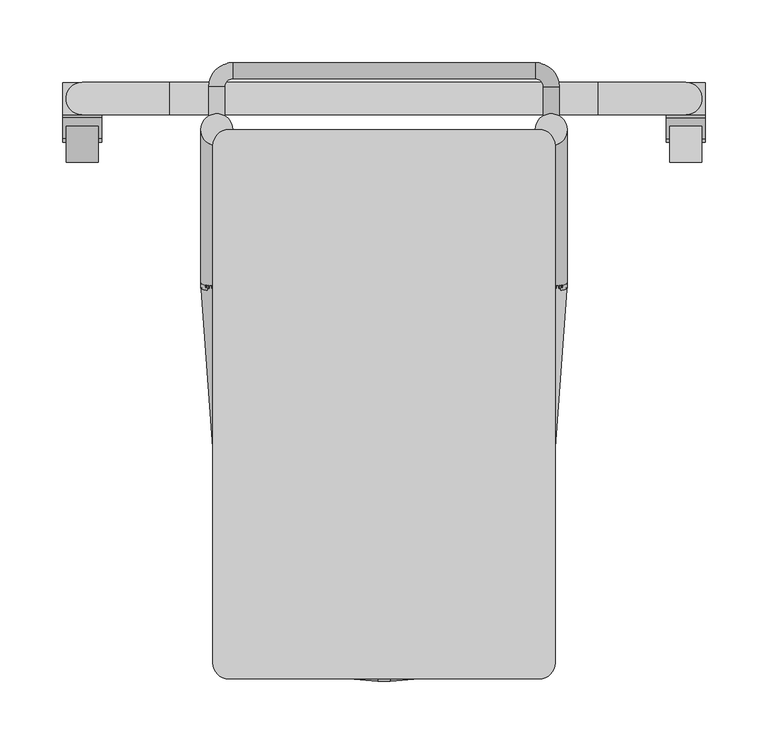
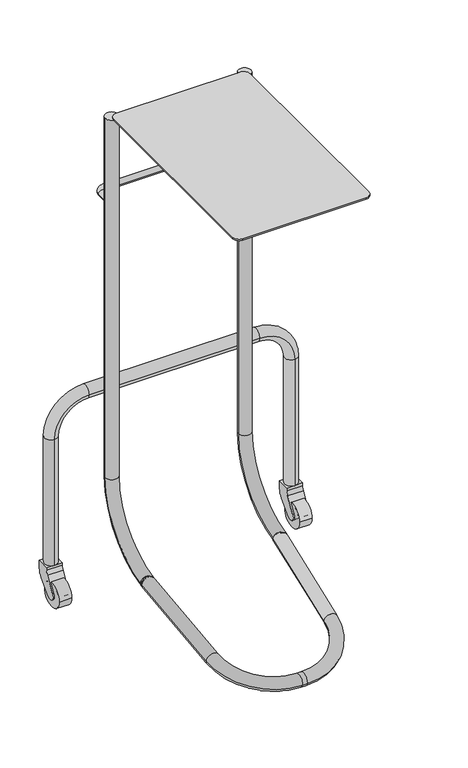
"""IFC4 building model written with IfcOpenShell, lengths in millimetres: proxy geometry, M8810 - Stand, Mayo : M8810 - Stand, Mayo."""

import ifcopenshell
import ifcopenshell.guid

model = None  # the IFC model being written
_history = None  # IfcOwnerHistory: only IFC2X3 demands one
_inside = {}  # id of a spatial element -> (the spatial element, [elements in it])
_under = {}  # id of a project, library or spatial element -> (it, [spatial elements below it])
_declared = {}  # id of a project -> (the project, [libraries it declares])
_typed = {}  # id of a type object -> (the type object, [elements of that type])
_made_of = {}  # id of a material, layer set ... -> (it, [elements and type objects made of it])


def new_model(schema):
    """Start an empty IFC model of exactly this schema.

    Asked for "IFC4X3", IfcOpenShell would pick the latest addendum, in which some entities
    have other attributes; the version numbers below select the first issue.
    IFC2X3 requires an IfcOwnerHistory on every rooted entity: one is made here for all.
    """
    global model, _history
    if schema == "IFC4X3":
        model = ifcopenshell.file(schema_version=(4, 3, 0, 0))
    else:
        model = ifcopenshell.file(schema=schema)
    _inside.clear()
    _under.clear()
    _declared.clear()
    _typed.clear()
    _made_of.clear()
    _history = None
    if model.schema == "IFC2X3":
        org = make("IfcOrganization", Name="unknown")
        user = make(
            "IfcPersonAndOrganization",
            ThePerson=make("IfcPerson", FamilyName="unknown"),
            TheOrganization=org,
        )
        app = make(
            "IfcApplication",
            ApplicationDeveloper=org,
            Version="unknown",
            ApplicationFullName="unknown",
            ApplicationIdentifier="unknown",
        )
        _history = make(
            "IfcOwnerHistory",
            OwningUser=user,
            OwningApplication=app,
            ChangeAction="ADDED",
            CreationDate=0,
        )
    return model


def make(cls, **values):
    """One entity of the class cls with the attributes given. An attribute that is None is left unset."""
    return model.create_entity(
        cls, **{name: value for name, value in values.items() if value is not None}
    )


def rooted(cls, **values):
    """An entity with a GlobalId (a new one), such as an element, a storey or a relation."""
    return make(cls, GlobalId=ifcopenshell.guid.new(), OwnerHistory=_history, **values)


def si_unit(unit_type, name, prefix=None):
    """IfcSIUnit, for example si_unit("LENGTHUNIT", "METRE", prefix="MILLI")."""
    return make("IfcSIUnit", UnitType=unit_type, Prefix=prefix, Name=name)


def assignment(units):
    """IfcUnitAssignment: the units of a project."""
    return None if units is None else make("IfcUnitAssignment", Units=units)


def point(xyz):
    """IfcCartesianPoint."""
    return None if xyz is None else make("IfcCartesianPoint", Coordinates=xyz)


def direction(xyz):
    """IfcDirection."""
    return None if xyz is None else make("IfcDirection", DirectionRatios=xyz)


def frame(location, z_axis=None, x_axis=None):
    """IfcAxis2Placement3D, a coordinate frame: its origin and axes. An axis left out is left unset."""
    return make(
        "IfcAxis2Placement3D",
        Location=point(location),
        Axis=direction(z_axis),
        RefDirection=direction(x_axis),
    )


def frame_2d(location, x_axis=None):
    """IfcAxis2Placement2D, a coordinate frame in the plane: its origin and x axis."""
    return make(
        "IfcAxis2Placement2D", Location=point(location), RefDirection=direction(x_axis)
    )


def origin():
    """The frame at (0, 0, 0) with its axes left unset."""
    return frame((0.0, 0.0, 0.0))


def place(relative_to, where):
    """IfcLocalPlacement: puts the frame where relative to a parent placement (None: the world)."""
    return make(
        "IfcLocalPlacement", PlacementRelTo=relative_to, RelativePlacement=where
    )


def context(
    kind, dimensions, precision=None, world=None, true_north=None, identifier=None
):
    """IfcGeometricRepresentationContext, for example the 3D "Model" context."""
    return make(
        "IfcGeometricRepresentationContext",
        ContextIdentifier=identifier,
        ContextType=kind,
        CoordinateSpaceDimension=dimensions,
        Precision=precision,
        WorldCoordinateSystem=world,
        TrueNorth=true_north,
    )


def project(units=None, contexts=None):
    """IfcProject with its units and contexts."""
    return rooted(
        "IfcProject",
        Name="project",
        RepresentationContexts=contexts,
        UnitsInContext=assignment(units),
    )


def spatial(cls, under=None, at=None, **own):
    """A site, building, storey or space (cls), placed at a placement, below another one or the project."""
    s = rooted(cls, ObjectPlacement=at, **own)
    if under is not None:
        _under.setdefault(under.id(), (under, []))[1].append(s)
    return s


def polyline(points):
    """IfcPolyline through the points."""
    return make("IfcPolyline", Points=[point(p) for p in points])


def circle_curve(where, radius):
    """IfcCircle in the frame where."""
    return make("IfcCircle", Position=where, Radius=radius)


def ellipse_curve(where, semi_axis1, semi_axis2):
    """IfcEllipse in the frame where."""
    return make(
        "IfcEllipse", Position=where, SemiAxis1=semi_axis1, SemiAxis2=semi_axis2
    )


def trimmed(basis, trim1, trim2, sense, master):
    """IfcTrimmedCurve: the piece of a basis curve between two trims."""
    return make(
        "IfcTrimmedCurve",
        BasisCurve=basis,
        Trim1=trim1,
        Trim2=trim2,
        SenseAgreement=sense,
        MasterRepresentation=master,
    )


def segment(curve, same_sense, transition):
    """IfcCompositeCurveSegment."""
    return make(
        "IfcCompositeCurveSegment",
        Transition=transition,
        SameSense=same_sense,
        ParentCurve=curve,
    )


def composite_curve(segments, self_intersect=None):
    """IfcCompositeCurve: segments joined end to end."""
    return make("IfcCompositeCurve", Segments=segments, SelfIntersect=self_intersect)


def outline(outer, holes=None, kind="AREA"):
    """IfcArbitraryClosedProfileDef: a profile drawn as a closed curve; with holes, ...WithVoids."""
    if holes is None:
        return make("IfcArbitraryClosedProfileDef", ProfileType=kind, OuterCurve=outer)
    return make(
        "IfcArbitraryProfileDefWithVoids",
        ProfileType=kind,
        OuterCurve=outer,
        InnerCurves=holes,
    )


def extrude(swept, where, along, depth):
    """IfcExtrudedAreaSolid: the profile swept, set in the frame where, extruded along a direction by depth."""
    return make(
        "IfcExtrudedAreaSolid",
        SweptArea=swept,
        Position=where,
        ExtrudedDirection=direction(along),
        Depth=depth,
    )


def shape(context_of_items, identifier, shape_type, items):
    """IfcShapeRepresentation: the items that make up one representation, for example the "Body"."""
    return make(
        "IfcShapeRepresentation",
        ContextOfItems=context_of_items,
        RepresentationIdentifier=identifier,
        RepresentationType=shape_type,
        Items=items,
    )


def source(mapping_origin, context_of_items, identifier, shape_type, items):
    """IfcRepresentationMap: a shape defined once, which mapped items show again and again."""
    return make(
        "IfcRepresentationMap",
        MappingOrigin=mapping_origin,
        MappedRepresentation=shape(context_of_items, identifier, shape_type, items),
    )


def transform(
    local_origin,
    x_axis=None,
    y_axis=None,
    z_axis=None,
    scale=None,
    scale2=None,
    scale3=None,
    uniform=True,
):
    """IfcCartesianTransformationOperator3D, or its non-uniform kind. x_axis, y_axis, z_axis: its Axis1, 2, 3."""
    if uniform:
        return make(
            "IfcCartesianTransformationOperator3D",
            Axis1=direction(x_axis),
            Axis2=direction(y_axis),
            LocalOrigin=point(local_origin),
            Scale=scale,
            Axis3=direction(z_axis),
        )
    return make(
        "IfcCartesianTransformationOperator3DnonUniform",
        Axis1=direction(x_axis),
        Axis2=direction(y_axis),
        LocalOrigin=point(local_origin),
        Scale=scale,
        Axis3=direction(z_axis),
        Scale2=scale2,
        Scale3=scale3,
    )


def mapped(mapping_source, mapping_target):
    """IfcMappedItem: shows the shape of a source again, moved by a transform."""
    return make(
        "IfcMappedItem", MappingSource=mapping_source, MappingTarget=mapping_target
    )


def made_of(thing, what):
    """Note that an element or type object is made of a material, layer set ...; save() writes the relation."""
    if what is not None:
        _made_of.setdefault(what.id(), (what, []))[1].append(thing)
    return thing


def element(
    cls,
    number,
    at=None,
    inside=None,
    cuts=None,
    type_object=None,
    material=None,
    context=None,
    identifier="Body",
    shape_type=None,
    held_by="IfcProductDefinitionShape",
    body=None,
    shapes=None,
    **own,
):
    """One element of the class cls, such as IfcWall. Its Tag is "e" and its number.

    at: its placement. inside: the storey or other place that contains it. cuts: it is an
    opening in that element (IfcRelVoidsElement). A single representation is given by context,
    identifier, shape_type and body (its items); several are given by shapes. held_by: the class
    of the entity that holds the representations. save() writes the other relations.
    """
    e = rooted(cls, Tag="e%d" % number, ObjectPlacement=at, **own)
    if body is not None:
        shapes = [shape(context, identifier, shape_type, body)]
    if shapes is not None:
        e.Representation = make(held_by, Representations=shapes)
    if inside is not None:
        _inside.setdefault(inside.id(), (inside, []))[1].append(e)
    if cuts is not None:
        rooted(
            "IfcRelVoidsElement", RelatingBuildingElement=cuts, RelatedOpeningElement=e
        )
    if type_object is not None:
        _typed.setdefault(type_object.id(), (type_object, []))[1].append(e)
    return made_of(e, material)


def aggregate(whole, parts):
    """IfcRelAggregates: a whole, such as a stair, and the parts it consists of."""
    return rooted("IfcRelAggregates", RelatingObject=whole, RelatedObjects=parts)


def save(model, path):
    """Write the relations noted so far, then the file.

    IfcRelAggregates (storeys below a building ...), IfcRelContainedInSpatialStructure (elements
    in a storey), IfcRelDefinesByType, IfcRelAssociatesMaterial and IfcRelDeclares: one each for
    every whole, place, type object, material and project.
    """
    for whole, parts in _under.values():
        aggregate(whole, parts)
    for where, things in _inside.values():
        rooted(
            "IfcRelContainedInSpatialStructure",
            RelatedElements=things,
            RelatingStructure=where,
        )
    for kind, things in _typed.values():
        rooted("IfcRelDefinesByType", RelatedObjects=things, RelatingType=kind)
    for what, things in _made_of.values():
        rooted("IfcRelAssociatesMaterial", RelatedObjects=things, RelatingMaterial=what)
    for by, libraries in _declared.values():
        rooted("IfcRelDeclares", RelatingContext=by, RelatedDefinitions=libraries)
    model.write(path)


def plane_surface(at):
    """IfcPlane: the flat surface through the origin of the frame at, square to its z axis."""
    return make("IfcPlane", Position=at)


def cylinder_surface(at, radius):
    """IfcCylindricalSurface: all points at the distance radius from the z axis of the frame at."""
    return make("IfcCylindricalSurface", Position=at, Radius=radius)


def revolved_surface(curve, axis_point, axis_direction):
    """IfcSurfaceOfRevolution: the curve turned about the line through axis_point along axis_direction."""
    return make(
        "IfcSurfaceOfRevolution",
        SweptCurve=make("IfcArbitraryOpenProfileDef", ProfileType="CURVE", Curve=curve),
        AxisPosition=make("IfcAxis1Placement", Location=point(axis_point), Axis=direction(axis_direction)),
    )


def advanced_brep(points, edges, surfaces, faces):
    """IfcAdvancedBrep: a solid bounded by faces that lie on surfaces and meet in shared edges.

    An edge is (start, end): straight between two places in points (the first is 0);
    or (start, end, curve); or (start, end, curve, False) where it runs against its curve.
    A face is (place in surfaces, loops), or (place, loops, False) where it looks against
    its surface's normal. A loop lists edges by number (the first is 1), with a minus sign
    where the edge is run from its end to its start. The first loop is the outer one.
    """
    corners = [point(p) for p in points]
    vertices = [make("IfcVertexPoint", VertexGeometry=c) for c in corners]
    made = []
    for start, end, *more in edges:
        made.append(
            make(
                "IfcEdgeCurve",
                EdgeStart=vertices[start],
                EdgeEnd=vertices[end],
                EdgeGeometry=more[0] if more else make("IfcPolyline", Points=[corners[start], corners[end]]),
                SameSense=more[1] if len(more) > 1 else True,
            )
        )
    hull = []
    for where, loops, *sense in faces:
        bounds = []
        for j, loop in enumerate(loops):
            ring = [make("IfcOrientedEdge", EdgeElement=made[abs(k) - 1], Orientation=k > 0) for k in loop]
            bounds.append(
                make(
                    "IfcFaceOuterBound" if j == 0 else "IfcFaceBound",
                    Bound=make("IfcEdgeLoop", EdgeList=ring),
                    Orientation=True,
                )
            )
        hull.append(make("IfcAdvancedFace", Bounds=bounds, FaceSurface=surfaces[where], SameSense=sense[0] if sense else True))
    return make("IfcAdvancedBrep", Outer=make("IfcClosedShell", CfsFaces=hull))


def specialty_equipment_49bd53c9(model_context):
    return source(origin(), model_context, "Body", "SolidModel", [
        advanced_brep(
        [(-126.6890783, 210.8754424, 812.8), (-139.3890783, 210.8754424, 812.8), (-126.6890783, 236.2754424, 812.8), (-139.3890783, 236.2754424, 812.8), (-120.3390783, 255.3254424, 812.8), (-120.3390783, 242.6254424, 812.8), (120.9609217, 242.6254424, 812.8), (120.9609217, 255.3254424, 812.8), (140.0109217, 236.2754424, 812.8), (127.3109217, 236.2754424, 812.8), (127.3109217, 210.8754424, 812.8), (140.0109217, 210.8754424, 812.8)],
        [
            (0, 1, circle_curve(frame((-133.0390783, 210.8754424, 812.8), z_axis=(0.0, -1.0, 0.0), x_axis=(-1.0, 0.0, 0.0)), 6.35)),
            (1, 0, circle_curve(frame((-133.0390783, 210.8754424, 812.8), z_axis=(0.0, -1.0, 0.0), x_axis=(-1.0, 0.0, 0.0)), 6.35)),
            (0, 2),
            (2, 3, circle_curve(frame((-133.0390783, 236.2754424, 812.8), z_axis=(0.0, -1.0, 0.0), x_axis=(-1.0, 0.0, 0.0)), 6.35)),
            (3, 1),
            (3, 2, circle_curve(frame((-133.0390783, 236.2754424, 812.8), z_axis=(0.0, -1.0, 0.0), x_axis=(-1.0, 0.0, 0.0)), 6.35)),
            (4, 3, circle_curve(frame((-120.3390783, 236.2754424, 812.8), z_axis=(0.0, 0.0, 1.0), x_axis=(-1.0, 0.0, 0.0)), 19.05)),
            (2, 5, circle_curve(frame((-120.3390783, 236.2754424, 812.8), z_axis=(0.0, 0.0, -1.0), x_axis=(-1.0, 0.0, 0.0)), 6.35)),
            (5, 4, circle_curve(frame((-120.3390783, 248.9754424, 812.8), z_axis=(-1.0, 0.0, 0.0), x_axis=(0.0, 1.0, 0.0)), 6.35)),
            (4, 5, circle_curve(frame((-120.3390783, 248.9754424, 812.8), z_axis=(-1.0, 0.0, 0.0), x_axis=(0.0, 1.0, 0.0)), 6.35)),
            (5, 6),
            (6, 7, circle_curve(frame((120.9609217, 248.9754424, 812.8), z_axis=(-1.0, 0.0, 0.0), x_axis=(0.0, 1.0, 0.0)), 6.35)),
            (7, 4),
            (7, 6, circle_curve(frame((120.9609217, 248.9754424, 812.8), z_axis=(-1.0, 0.0, 0.0), x_axis=(0.0, 1.0, 0.0)), 6.35)),
            (8, 7, circle_curve(frame((120.9609217, 236.2754424, 812.8), z_axis=(0.0, 0.0, 1.0), x_axis=(0.0, 1.0, 0.0)), 19.05)),
            (6, 9, circle_curve(frame((120.9609217, 236.2754424, 812.8), z_axis=(0.0, 0.0, -1.0), x_axis=(0.0, 1.0, 0.0)), 6.35)),
            (9, 8, circle_curve(frame((133.6609217, 236.2754424, 812.8), z_axis=(0.0, 1.0, 0.0), x_axis=(1.0, 0.0, 0.0)), 6.35)),
            (8, 9, circle_curve(frame((133.6609217, 236.2754424, 812.8), z_axis=(0.0, 1.0, 0.0), x_axis=(1.0, 0.0, 0.0)), 6.35)),
            (10, 11, circle_curve(frame((133.6609217, 210.8754424, 812.8), z_axis=(0.0, -1.0, 0.0), x_axis=(1.0, 0.0, 0.0)), 6.35)),
            (11, 10, circle_curve(frame((133.6609217, 210.8754424, 812.8), z_axis=(0.0, -1.0, 0.0), x_axis=(1.0, 0.0, 0.0)), 6.35)),
            (9, 10),
            (11, 8),
        ],
        [
            plane_surface(frame((-133.0390783, 210.8754424, 0.0), z_axis=(0.0, -1.0, 0.0), x_axis=(0.0, 0.0, 1.0))),
            cylinder_surface(frame((-133.0390783, 210.8754424, 812.8), z_axis=(0.0, -1.0, 0.0), x_axis=(-1.0, 0.0, 0.0)), 6.35),
            revolved_surface(trimmed(ellipse_curve(frame((-133.0390783, 236.2754424, 812.8), z_axis=(0.0, -1.0, 0.0), x_axis=(-1.0, 0.0, 0.0)), 6.35, 6.35), [point((-126.6890783, 236.2754424, 812.8))], [point((-139.3890783, 236.2754424, 812.8))], True, "CARTESIAN"), (-120.3390783, 236.2754424, 0.0), (0.0, 0.0, -1.0)),
            revolved_surface(trimmed(ellipse_curve(frame((-133.0390783, 236.2754424, 812.8), z_axis=(0.0, -1.0, 0.0), x_axis=(-1.0, 0.0, 0.0)), 6.35, 6.35), [point((-139.3890783, 236.2754424, 812.8))], [point((-126.6890783, 236.2754424, 812.8))], True, "CARTESIAN"), (-120.3390783, 236.2754424, 0.0), (0.0, 0.0, -1.0)),
            cylinder_surface(frame((-120.3390783, 248.9754424, 812.8), z_axis=(-1.0, 0.0, 0.0), x_axis=(0.0, 1.0, 0.0)), 6.35),
            revolved_surface(trimmed(ellipse_curve(frame((120.9609217, 248.9754424, 812.8), z_axis=(-1.0, 0.0, 0.0), x_axis=(0.0, 1.0, 0.0)), 6.35, 6.35), [point((120.9609217, 242.6254424, 812.8))], [point((120.9609217, 255.3254424, 812.8))], True, "CARTESIAN"), (120.9609217, 236.2754424, 0.0), (0.0, 0.0, -1.0)),
            revolved_surface(trimmed(ellipse_curve(frame((120.9609217, 248.9754424, 812.8), z_axis=(-1.0, 0.0, 0.0), x_axis=(0.0, 1.0, 0.0)), 6.35, 6.35), [point((120.9609217, 255.3254424, 812.8))], [point((120.9609217, 242.6254424, 812.8))], True, "CARTESIAN"), (120.9609217, 236.2754424, 0.0), (0.0, 0.0, -1.0)),
            plane_surface(frame((133.6609217, 210.8754424, 0.0), z_axis=(0.0, -1.0, 0.0), x_axis=(0.0, 0.0, 1.0))),
            cylinder_surface(frame((133.6609217, 236.2754424, 812.8), z_axis=(0.0, 1.0, 0.0), x_axis=(1.0, 0.0, 0.0)), 6.35),
        ],
        [
            (0, [[1, 2]]),
            (1, [[-1, 3, 4, 5]]),
            (1, [[-2, -5, 6, -3]]),
            (2, [[7, -4, 8, 9]]),
            (3, [[-8, -6, -7, 10]]),
            (4, [[-9, 11, 12, 13]]),
            (4, [[-10, -13, 14, -11]]),
            (5, [[15, -12, 16, 17]]),
            (6, [[-16, -14, -15, 18]]),
            (7, [[19, 20]]),
            (8, [[-17, 21, -20, 22]]),
            (8, [[-18, -22, -19, -21]]),
        ],
    ),
        advanced_brep(
        [(241.1146411, 213.8046841, 76.2), (241.1146411, 239.7603256, 76.2), (241.1146411, 213.8046841, 342.9), (241.1146411, 239.7603256, 342.9), (171.2646411, 239.7603256, 412.75), (171.2646411, 213.8046841, 412.75), (-170.6427977, 213.8046841, 412.75), (-170.6427977, 239.7603256, 412.75), (-240.4927977, 239.7603256, 342.9), (-240.4927977, 213.8046841, 342.9), (-240.4927977, 213.8046841, 76.2), (-240.4927977, 239.7603256, 76.2)],
        [
            (0, 1, circle_curve(frame((241.1146411, 226.7825049, 76.2), z_axis=(0.0, 0.0, -1.0), x_axis=(0.0, 1.0, 0.0)), 12.9778207)),
            (1, 0, circle_curve(frame((241.1146411, 226.7825049, 76.2), z_axis=(0.0, 0.0, -1.0), x_axis=(0.0, 1.0, 0.0)), 12.9778207)),
            (0, 2),
            (2, 3, circle_curve(frame((241.1146411, 226.7825049, 342.9), z_axis=(0.0, 0.0, -1.0), x_axis=(0.0, 1.0, 0.0)), 12.9778207)),
            (3, 1),
            (3, 2, circle_curve(frame((241.1146411, 226.7825049, 342.9), z_axis=(0.0, 0.0, -1.0), x_axis=(0.0, 1.0, 0.0)), 12.9778207)),
            (4, 3, circle_curve(frame((171.2646411, 239.7603256, 342.9), z_axis=(0.0, 1.0, 0.0), x_axis=(1.0, 0.0, 0.0)), 69.85)),
            (2, 5, circle_curve(frame((171.2646411, 213.8046841, 342.9), z_axis=(0.0, -1.0, 0.0), x_axis=(1.0, 0.0, 0.0)), 69.85)),
            (5, 4, circle_curve(frame((171.2646411, 226.7825049, 412.75), z_axis=(1.0, 0.0, 0.0), x_axis=(0.0, 1.0, 0.0)), 12.9778207)),
            (4, 5, circle_curve(frame((171.2646411, 226.7825049, 412.75), z_axis=(1.0, 0.0, 0.0), x_axis=(0.0, 1.0, 0.0)), 12.9778207)),
            (5, 6),
            (6, 7, circle_curve(frame((-170.6427977, 226.7825049, 412.75), z_axis=(1.0, 0.0, 0.0), x_axis=(0.0, 1.0, 0.0)), 12.9778207)),
            (7, 4),
            (7, 6, circle_curve(frame((-170.6427977, 226.7825049, 412.75), z_axis=(1.0, 0.0, 0.0), x_axis=(0.0, 1.0, 0.0)), 12.9778207)),
            (8, 7, circle_curve(frame((-170.6427977, 239.7603256, 342.9), z_axis=(0.0, 1.0, 0.0), x_axis=(0.0, 0.0, 1.0)), 69.85)),
            (6, 9, circle_curve(frame((-170.6427977, 213.8046841, 342.9), z_axis=(0.0, -1.0, 0.0), x_axis=(0.0, 0.0, 1.0)), 69.85)),
            (9, 8, circle_curve(frame((-240.4927977, 226.7825049, 342.9), z_axis=(0.0, 0.0, 1.0), x_axis=(0.0, 1.0, 0.0)), 12.9778207)),
            (8, 9, circle_curve(frame((-240.4927977, 226.7825049, 342.9), z_axis=(0.0, 0.0, 1.0), x_axis=(0.0, 1.0, 0.0)), 12.9778207)),
            (10, 11, circle_curve(frame((-240.4927977, 226.7825049, 76.2), z_axis=(0.0, 0.0, -1.0), x_axis=(0.0, 1.0, 0.0)), 12.9778207)),
            (11, 10, circle_curve(frame((-240.4927977, 226.7825049, 76.2), z_axis=(0.0, 0.0, -1.0), x_axis=(0.0, 1.0, 0.0)), 12.9778207)),
            (9, 10),
            (11, 8),
        ],
        [
            plane_surface(frame((241.1146411, -17.2197448, 76.2), z_axis=(0.0, 0.0, -1.0), x_axis=(0.0, 1.0, 0.0))),
            cylinder_surface(frame((241.1146411, 226.7825049, 76.2), z_axis=(0.0, 0.0, -1.0), x_axis=(0.0, 1.0, 0.0)), 12.9778207),
            revolved_surface(trimmed(ellipse_curve(frame((241.1146411, 226.7825049, 342.9), z_axis=(0.0, 0.0, -1.0), x_axis=(0.0, 1.0, 0.0)), 12.9778207, 12.9778207), [point((241.1146411, 213.8046841, 342.9))], [point((241.1146411, 239.7603256, 342.9))], True, "CARTESIAN"), (171.2646411, -17.2197448, 342.9), (0.0, -1.0, 0.0)),
            revolved_surface(trimmed(ellipse_curve(frame((241.1146411, 226.7825049, 342.9), z_axis=(0.0, 0.0, -1.0), x_axis=(0.0, 1.0, 0.0)), 12.9778207, 12.9778207), [point((241.1146411, 239.7603256, 342.9))], [point((241.1146411, 213.8046841, 342.9))], True, "CARTESIAN"), (171.2646411, -17.2197448, 342.9), (0.0, -1.0, 0.0)),
            cylinder_surface(frame((171.2646411, 226.7825049, 412.75), z_axis=(1.0, 0.0, 0.0), x_axis=(0.0, 1.0, 0.0)), 12.9778207),
            revolved_surface(trimmed(ellipse_curve(frame((-170.6427977, 226.7825049, 412.75), z_axis=(1.0, 0.0, 0.0), x_axis=(0.0, 1.0, 0.0)), 12.9778207, 12.9778207), [point((-170.6427977, 213.8046841, 412.75))], [point((-170.6427977, 239.7603256, 412.75))], True, "CARTESIAN"), (-170.6427977, -17.2197448, 342.9), (0.0, -1.0, 0.0)),
            revolved_surface(trimmed(ellipse_curve(frame((-170.6427977, 226.7825049, 412.75), z_axis=(1.0, 0.0, 0.0), x_axis=(0.0, 1.0, 0.0)), 12.9778207, 12.9778207), [point((-170.6427977, 239.7603256, 412.75))], [point((-170.6427977, 213.8046841, 412.75))], True, "CARTESIAN"), (-170.6427977, -17.2197448, 342.9), (0.0, -1.0, 0.0)),
            plane_surface(frame((-240.4927977, -17.2197448, 76.2), z_axis=(0.0, 0.0, -1.0), x_axis=(0.0, 1.0, 0.0))),
            cylinder_surface(frame((-240.4927977, 226.7825049, 342.9), z_axis=(0.0, 0.0, 1.0), x_axis=(0.0, 1.0, 0.0)), 12.9778207),
        ],
        [
            (0, [[1, 2]]),
            (1, [[-1, 3, 4, 5]]),
            (1, [[-2, -5, 6, -3]]),
            (2, [[7, -4, 8, 9]]),
            (3, [[-8, -6, -7, 10]]),
            (4, [[-9, 11, 12, 13]]),
            (4, [[-10, -13, 14, -11]]),
            (5, [[15, -12, 16, 17]]),
            (6, [[-16, -14, -15, 18]]),
            (7, [[19, 20]]),
            (8, [[-17, 21, -20, 22]]),
            (8, [[-18, -22, -19, -21]]),
        ],
    ),
        extrude(outline(composite_curve([segment(trimmed(circle_curve(frame_2d((216.9079352, 59.8228937)), 22.6440422), [point((239.5519774, 59.8228937))], [point((232.5453683, 43.4453685))], False, "CARTESIAN"), True, "CONTINUOUS"), segment(polyline([(232.5453683, 43.4453685), (208.3430256, 19.2430257)]), True, "CONTINUOUS"), segment(trimmed(circle_curve(frame_2d((201.6078335, 25.9782178)), 9.525), [point((208.3430256, 19.2430257))], [point((194.8726414, 32.7134099))], False, "CARTESIAN"), True, "CONTINUOUS"), segment(polyline([(194.8726414, 32.7134099), (211.5132649, 61.5358153)]), True, "CONTINUOUS"), segment(trimmed(circle_curve(frame_2d((194.9390027, 71.1049701)), 19.1383095), [point((211.5132649, 61.5358153))], [point((214.0560132, 70.2023074))], True, "CARTESIAN"), True, "CONTINUOUS"), segment(polyline([(214.0560132, 70.2023074), (214.0560132, 76.2), (239.5519774, 76.2), (239.5519774, 59.8228937)]), True, "CONTINUOUS")], self_intersect=False)), frame((225.5357109, 0.0, 0.0), z_axis=(1.0, 0.0, 0.0), x_axis=(0.0, 1.0, 0.0)), (0.0, 0.0, 1.0), 31.1578605),
        extrude(outline(composite_curve([segment(trimmed(circle_curve(frame_2d((201.4519773, 25.4)), 25.4), [point((176.0519773, 25.4))], [point((226.8519773, 25.4))], False, "CARTESIAN"), True, "CONTINUOUS"), segment(trimmed(circle_curve(frame_2d((201.4519773, 25.4)), 25.4), [point((226.8519773, 25.4))], [point((176.0519773, 25.4))], False, "CARTESIAN"), True, "CONTINUOUS")], self_intersect=False)), frame((228.4777015, 0.0, 0.0), z_axis=(1.0, 0.0, 0.0), x_axis=(0.0, 1.0, 0.0)), (0.0, 0.0, 1.0), 25.4),
        extrude(outline(composite_curve([segment(trimmed(circle_curve(frame_2d((216.9079352, 59.8228937)), 22.6440422), [point((239.5519774, 59.8228937))], [point((232.5453683, 43.4453685))], False, "CARTESIAN"), True, "CONTINUOUS"), segment(polyline([(232.5453683, 43.4453685), (208.3430256, 19.2430257)]), True, "CONTINUOUS"), segment(trimmed(circle_curve(frame_2d((201.6078335, 25.9782178)), 9.525), [point((208.3430256, 19.2430257))], [point((194.8726414, 32.7134099))], False, "CARTESIAN"), True, "CONTINUOUS"), segment(polyline([(194.8726414, 32.7134099), (211.5132649, 61.5358153)]), True, "CONTINUOUS"), segment(trimmed(circle_curve(frame_2d((194.9390027, 71.1049701)), 19.1383095), [point((211.5132649, 61.5358153))], [point((214.0560132, 70.2023074))], True, "CARTESIAN"), True, "CONTINUOUS"), segment(polyline([(214.0560132, 70.2023074), (214.0560132, 76.2), (239.5519774, 76.2), (239.5519774, 59.8228937)]), True, "CONTINUOUS")], self_intersect=False)), frame((-256.071728, 0.0, 0.0), z_axis=(1.0, 0.0, 0.0), x_axis=(0.0, 1.0, 0.0)), (0.0, 0.0, 1.0), 31.1578605),
        extrude(outline(composite_curve([segment(trimmed(circle_curve(frame_2d((201.4519773, 25.4)), 25.4), [point((176.0519773, 25.4))], [point((226.8519773, 25.4))], False, "CARTESIAN"), True, "CONTINUOUS"), segment(trimmed(circle_curve(frame_2d((201.4519773, 25.4)), 25.4), [point((226.8519773, 25.4))], [point((176.0519773, 25.4))], False, "CARTESIAN"), True, "CONTINUOUS")], self_intersect=False)), frame((-253.2558581, 0.0, 0.0), z_axis=(1.0, 0.0, 0.0), x_axis=(0.0, 1.0, 0.0)), (0.0, 0.0, 1.0), 25.4),
        advanced_brep(
        [(-145.7081418, 79.7843699, 86.3661535), (-120.3700149, 81.5107728, 86.764725), (-131.1843024, -122.5928577, 39.643689), (-105.8461755, -120.8664548, 40.0422606), (-4.493668, -212.9568416, 18.7815195), (-4.493668, -237.7058412, 13.0677627), (5.1155113, -237.7058412, 13.0677627), (5.1155113, -212.9568416, 18.7815195), (106.4680188, -120.8664548, 40.0422606), (131.8061457, -122.5928577, 39.643689), (146.3299851, 79.7843699, 86.3661535), (120.9918582, 81.5107728, 86.764725)],
        [
            (0, 1, circle_curve(frame((-133.0390783, 80.6475713, 86.5654393), z_axis=(-0.0697564737441234, 0.9719965482790884, 0.22440308488147717), x_axis=(0.9975640502598245, 0.06796861984125109, 0.015691792316050647)), 12.7)),
            (1, 0, circle_curve(frame((-133.0390783, 80.6475713, 86.5654393), z_axis=(-0.0697564737441234, 0.9719965482790884, 0.22440308488147717), x_axis=(0.9975640502598245, 0.06796861984125109, 0.015691792316050647)), 12.7)),
            (0, 2),
            (2, 3, circle_curve(frame((-118.5152389, -121.7296563, 39.8429748), z_axis=(-0.0697564737441234, 0.9719965482790884, 0.22440308488147717), x_axis=(0.9975640502598245, 0.06796861984125109, 0.015691792316050647)), 12.7)),
            (3, 1),
            (3, 2, circle_curve(frame((-118.5152389, -121.7296563, 39.8429748), z_axis=(-0.0697564737441234, 0.9719965482790884, 0.22440308488147717), x_axis=(0.9975640502598245, 0.06796861984125109, 0.015691792316050647)), 12.7)),
            (4, 3, circle_curve(frame((-4.493668, -113.960843, 41.6365466), z_axis=(0.0, 0.22495105434385831, -0.9743700647852368), x_axis=(-0.9975640502598243, -0.06796861984125117, -0.015691792316050664)), 101.6)),
            (2, 5, circle_curve(frame((-4.493668, -113.960843, 41.6365466), z_axis=(0.0, -0.22495105434385831, 0.9743700647852368), x_axis=(-0.9975640502598243, -0.06796861984125117, -0.015691792316050664)), 127.0)),
            (5, 4, circle_curve(frame((-4.493668, -225.3313414, 15.9246411), z_axis=(-0.9999999999999999, 0.0, 0.0), x_axis=(0.0, 0.9743700647852367, 0.2249510543438583)), 12.7)),
            (4, 5, circle_curve(frame((-4.493668, -225.3313414, 15.9246411), z_axis=(-1.0, 0.0, 0.0), x_axis=(0.0, 0.9743700647852367, 0.22495105434385831)), 12.7)),
            (5, 6),
            (6, 7, circle_curve(frame((5.1155113, -225.3313414, 15.9246411), z_axis=(-1.0, 0.0, 0.0), x_axis=(0.0, 0.9743700647852369, 0.22495105434385834)), 12.7)),
            (7, 4),
            (7, 6, circle_curve(frame((5.1155113, -225.3313414, 15.9246411), z_axis=(-1.0, 0.0, 0.0), x_axis=(0.0, 0.9743700647852369, 0.22495105434385834)), 12.7)),
            (8, 7, circle_curve(frame((5.1155113, -113.960843, 41.6365466), z_axis=(0.0, 0.22495105434385831, -0.9743700647852368), x_axis=(0.0, -0.9743700647852368, -0.22495105434385831)), 101.6)),
            (6, 9, circle_curve(frame((5.1155113, -113.960843, 41.6365466), z_axis=(0.0, -0.22495105434385831, 0.9743700647852368), x_axis=(0.0, -0.9743700647852368, -0.22495105434385831)), 127.0)),
            (9, 8, circle_curve(frame((119.1370823, -121.7296563, 39.8429748), z_axis=(-0.06975647374412788, -0.971996548279088, -0.22440308488147714), x_axis=(-0.9975640502598241, 0.06796861984125566, 0.015691792316050824)), 12.7)),
            (8, 9, circle_curve(frame((119.1370823, -121.7296563, 39.8429748), z_axis=(-0.06975647374412833, -0.971996548279088, -0.22440308488147714), x_axis=(-0.9975640502598241, 0.06796861984125609, 0.01569179231605092)), 12.7)),
            (10, 11, circle_curve(frame((133.6609217, 80.6475713, 86.5654393), z_axis=(0.06975647374412713, 0.9719965482790881, 0.22440308488147723), x_axis=(-0.9975640502598242, 0.06796861984125492, 0.015691792316050664)), 12.7)),
            (11, 10, circle_curve(frame((133.6609217, 80.6475713, 86.5654393), z_axis=(0.06975647374412713, 0.9719965482790881, 0.22440308488147723), x_axis=(-0.9975640502598242, 0.06796861984125492, 0.015691792316050664)), 12.7)),
            (9, 10),
            (11, 8),
        ],
        [
            plane_surface(frame((-133.0390783, 80.6475713, 86.5654393), z_axis=(-0.0697564737441234, 0.9719965482790884, 0.22440308488147717), x_axis=(0.0, -0.22495105434385831, 0.9743700647852368))),
            cylinder_surface(frame((-133.0390783, 80.6475713, 86.5654393), z_axis=(-0.0697564737441234, 0.9719965482790884, 0.22440308488147717), x_axis=(0.9975640502598245, 0.06796861984125109, 0.015691792316050647)), 12.7),
            revolved_surface(trimmed(ellipse_curve(frame((-118.5152389, -121.7296563, 39.8429748), z_axis=(-0.06975647374412344, 0.9719965482790882, 0.22440308488147712), x_axis=(0.9975640502598243, 0.06796861984125113, 0.01569179231605066)), 12.7, 12.7), [point((-131.1843024, -122.5928577, 39.643689))], [point((-105.8461755, -120.8664548, 40.0422606))], True, "CARTESIAN"), (-4.493668, -113.960843, 41.6365466), (0.0, -0.22495105434385831, 0.9743700647852368)),
            revolved_surface(trimmed(ellipse_curve(frame((-118.5152389, -121.7296563, 39.8429748), z_axis=(-0.06975647374412344, 0.9719965482790882, 0.22440308488147712), x_axis=(0.9975640502598243, 0.06796861984125113, 0.01569179231605066)), 12.7, 12.7), [point((-105.8461755, -120.8664548, 40.0422606))], [point((-131.1843024, -122.5928577, 39.643689))], True, "CARTESIAN"), (-4.493668, -113.960843, 41.6365466), (0.0, -0.22495105434385831, 0.9743700647852368)),
            cylinder_surface(frame((-4.493668, -225.3313414, 15.9246411), z_axis=(-1.0000000000000002, 0.0, 0.0), x_axis=(0.0, 0.9743700647852369, 0.22495105434385834)), 12.7),
            revolved_surface(trimmed(ellipse_curve(frame((5.1155113, -225.3313414, 15.9246411), z_axis=(-1.0, 0.0, 0.0), x_axis=(0.0, 0.9743700647852368, 0.22495105434385831)), 12.7, 12.7), [point((5.1155113, -237.7058412, 13.0677627))], [point((5.1155113, -212.9568416, 18.7815195))], True, "CARTESIAN"), (5.1155113, -113.960843, 41.6365466), (0.0, -0.22495105434385831, 0.9743700647852368)),
            revolved_surface(trimmed(ellipse_curve(frame((5.1155113, -225.3313414, 15.9246411), z_axis=(-1.0, 0.0, 0.0), x_axis=(0.0, 0.9743700647852368, 0.22495105434385831)), 12.7, 12.7), [point((5.1155113, -212.9568416, 18.7815195))], [point((5.1155113, -237.7058412, 13.0677627))], True, "CARTESIAN"), (5.1155113, -113.960843, 41.6365466), (0.0, -0.22495105434385831, 0.9743700647852368)),
            plane_surface(frame((133.6609217, 80.6475713, 86.5654393), z_axis=(0.06975647374412708, 0.971996548279088, 0.22440308488147714), x_axis=(0.0, -0.22495105434385834, 0.9743700647852368))),
            cylinder_surface(frame((119.1370823, -121.7296563, 39.8429748), z_axis=(-0.06975647374412713, -0.9719965482790881, -0.22440308488147723), x_axis=(-0.9975640502598242, 0.06796861984125492, 0.015691792316050664)), 12.7),
        ],
        [
            (0, [[1, 2]]),
            (1, [[-1, 3, 4, 5]]),
            (1, [[-2, -5, 6, -3]]),
            (2, [[7, -4, 8, 9]]),
            (3, [[-8, -6, -7, 10]]),
            (4, [[-9, 11, 12, 13]]),
            (4, [[-10, -13, 14, -11]]),
            (5, [[15, -12, 16, 17]]),
            (6, [[-16, -14, -15, 18]]),
            (7, [[19, 20]]),
            (8, [[-17, 21, -20, 22]]),
            (8, [[-18, -22, -19, -21]]),
        ],
    ),
        advanced_brep(
        [(146.3609217, 201.8552552, 996.6409151), (120.9609217, 201.8552552, 996.6409151), (146.3609217, 201.8552552, 235.8329339), (120.9609217, 201.8552552, 235.8329339), (146.3609217, 75.5574845, 85.6848949), (120.9609217, 75.5574845, 85.6848949)],
        [
            (0, 1, circle_curve(frame((133.6609217, 201.8552552, 996.6409151), z_axis=(0.0, 0.0, 1.0), x_axis=(-1.0, 0.0, 0.0)), 12.7)),
            (1, 0, circle_curve(frame((133.6609217, 201.8552552, 996.6409151), z_axis=(0.0, 0.0, 1.0), x_axis=(-1.0, 0.0, 0.0)), 12.7)),
            (0, 2),
            (2, 3, circle_curve(frame((133.6609217, 201.8552552, 235.8329339), z_axis=(0.0, 0.0, 1.0), x_axis=(-1.0, 0.0, 0.0)), 12.7)),
            (3, 1),
            (3, 2, circle_curve(frame((133.6609217, 201.8552552, 235.8329339), z_axis=(0.0, 0.0, 1.0), x_axis=(-1.0, 0.0, 0.0)), 12.7)),
            (4, 5, circle_curve(frame((133.6609217, 75.5574845, 85.6848949), z_axis=(0.0, -0.9852233532397917, -0.1712744704587949), x_axis=(-1.0, 0.0, 0.0)), 12.7)),
            (5, 4, circle_curve(frame((133.6609217, 75.5574845, 85.6848949), z_axis=(0.0, -0.9852233532397917, -0.1712744704587949), x_axis=(-1.0, 0.0, 0.0)), 12.7)),
            (5, 3, circle_curve(frame((120.9609217, 49.4552552, 235.8329339), z_axis=(1.0, 0.0, 0.0), x_axis=(0.0, 1.0, 0.0)), 152.4)),
            (2, 4, circle_curve(frame((146.3609217, 49.4552552, 235.8329339), z_axis=(-1.0, 0.0, 0.0), x_axis=(0.0, 1.0, 0.0)), 152.4)),
        ],
        [
            plane_surface(frame((0.3109217, 201.8552552, 996.6409151), z_axis=(0.0, 0.0, 1.0), x_axis=(-1.0, 0.0, 0.0))),
            cylinder_surface(frame((133.6609217, 201.8552552, 996.6409151), z_axis=(0.0, 0.0, 1.0), x_axis=(-1.0, 0.0, 0.0)), 12.7),
            plane_surface(frame((0.3109217, 75.5574845, 85.6848949), z_axis=(0.0, -0.9852233532397917, -0.17127447045879493), x_axis=(-1.0, 0.0, 0.0))),
            revolved_surface(trimmed(ellipse_curve(frame((133.6609217, 201.8552552, 235.8329339), z_axis=(0.0, 0.0, 1.0), x_axis=(-1.0, 0.0, 0.0)), 12.7, 12.7), [point((146.3609217, 201.8552552, 235.8329339))], [point((120.9609217, 201.8552552, 235.8329339))], True, "CARTESIAN"), (0.3109217, 49.4552552, 235.8329339), (-1.0, 0.0, 0.0)),
            revolved_surface(trimmed(ellipse_curve(frame((133.6609217, 201.8552552, 235.8329339), z_axis=(0.0, 0.0, 1.0), x_axis=(-1.0, 0.0, 0.0)), 12.7, 12.7), [point((120.9609217, 201.8552552, 235.8329339))], [point((146.3609217, 201.8552552, 235.8329339))], True, "CARTESIAN"), (0.3109217, 49.4552552, 235.8329339), (-1.0, 0.0, 0.0)),
        ],
        [
            (0, [[1, 2]]),
            (1, [[-1, 3, 4, 5]]),
            (1, [[-2, -5, 6, -3]]),
            (2, [[7, 8]]),
            (3, [[9, -4, 10, -8]]),
            (4, [[-10, -6, -9, -7]]),
        ],
    ),
        advanced_brep(
        [(-145.7390783, 201.8552552, 996.6409151), (-120.3390783, 201.8552552, 996.6409151), (-145.7390783, 201.8552552, 235.8329339), (-120.3390783, 201.8552552, 235.8329339), (-145.7390783, 75.5574845, 85.6848949), (-120.3390783, 75.5574845, 85.6848949)],
        [
            (0, 1, circle_curve(frame((-133.0390783, 201.8552552, 996.6409151), z_axis=(0.0, 0.0, 1.0), x_axis=(1.0, 0.0, 0.0)), 12.7)),
            (1, 0, circle_curve(frame((-133.0390783, 201.8552552, 996.6409151), z_axis=(0.0, 0.0, 1.0), x_axis=(1.0, 0.0, 0.0)), 12.7)),
            (0, 2),
            (2, 3, circle_curve(frame((-133.0390783, 201.8552552, 235.8329339), z_axis=(0.0, 0.0, 1.0), x_axis=(1.0, 0.0, 0.0)), 12.7)),
            (3, 1),
            (3, 2, circle_curve(frame((-133.0390783, 201.8552552, 235.8329339), z_axis=(0.0, 0.0, 1.0), x_axis=(1.0, 0.0, 0.0)), 12.7)),
            (4, 5, circle_curve(frame((-133.0390783, 75.5574845, 85.6848949), z_axis=(0.0, -0.9852233532397917, -0.1712744704587949), x_axis=(1.0, 0.0, 0.0)), 12.7)),
            (5, 4, circle_curve(frame((-133.0390783, 75.5574845, 85.6848949), z_axis=(0.0, -0.9852233532397917, -0.1712744704587949), x_axis=(1.0, 0.0, 0.0)), 12.7)),
            (5, 3, circle_curve(frame((-120.3390783, 49.4552552, 235.8329339), z_axis=(1.0, 0.0, 0.0), x_axis=(0.0, 1.0, 0.0)), 152.4)),
            (2, 4, circle_curve(frame((-145.7390783, 49.4552552, 235.8329339), z_axis=(-1.0, 0.0, 0.0), x_axis=(0.0, 1.0, 0.0)), 152.4)),
        ],
        [
            plane_surface(frame((0.3109217, 201.8552552, 996.6409151), z_axis=(0.0, 0.0, 1.0), x_axis=(1.0, 0.0, 0.0))),
            cylinder_surface(frame((-133.0390783, 201.8552552, 996.6409151), z_axis=(0.0, 0.0, 1.0), x_axis=(1.0, 0.0, 0.0)), 12.7),
            plane_surface(frame((0.3109217, 75.5574845, 85.6848949), z_axis=(0.0, -0.9852233532397917, -0.17127447045879493), x_axis=(1.0, 0.0, 0.0))),
            revolved_surface(trimmed(ellipse_curve(frame((-133.0390783, 201.8552552, 235.8329339), z_axis=(0.0, 0.0, 1.0), x_axis=(1.0, 0.0, 0.0)), 12.7, 12.7), [point((-145.7390783, 201.8552552, 235.8329339))], [point((-120.3390783, 201.8552552, 235.8329339))], True, "CARTESIAN"), (0.3109217, 49.4552552, 235.8329339), (-1.0, 0.0, 0.0)),
            revolved_surface(trimmed(ellipse_curve(frame((-133.0390783, 201.8552552, 235.8329339), z_axis=(0.0, 0.0, 1.0), x_axis=(1.0, 0.0, 0.0)), 12.7, 12.7), [point((-120.3390783, 201.8552552, 235.8329339))], [point((-145.7390783, 201.8552552, 235.8329339))], True, "CARTESIAN"), (0.3109217, 49.4552552, 235.8329339), (-1.0, 0.0, 0.0)),
        ],
        [
            (0, [[1, 2]]),
            (1, [[-1, 3, 4, 5]]),
            (1, [[-2, -5, 6, -3]]),
            (2, [[7, 8]]),
            (3, [[9, -4, 10, -8]]),
            (4, [[-10, -6, -9, -7]]),
        ],
    ),
        extrude(outline(composite_curve([segment(trimmed(circle_curve(frame_2d((-123.5140783, 189.1552552)), 12.7), [point((-136.2140783, 189.1552552))], [point((-123.5140783, 201.8552552))], False, "CARTESIAN"), True, "CONTINUOUS"), segment(polyline([(-123.5140783, 201.8552552), (124.1359217, 201.8552552)]), True, "CONTINUOUS"), segment(trimmed(circle_curve(frame_2d((124.1359217, 189.1552552)), 12.7), [point((124.1359217, 201.8552552))], [point((136.8359217, 189.1552552))], False, "CARTESIAN"), True, "CONTINUOUS"), segment(polyline([(136.8359217, 189.1552552), (136.8359217, -223.5947448)]), True, "CONTINUOUS"), segment(trimmed(circle_curve(frame_2d((124.1359217, -223.5947448)), 12.7), [point((136.8359217, -223.5947448))], [point((124.1359217, -236.2947448))], False, "CARTESIAN"), True, "CONTINUOUS"), segment(polyline([(124.1359217, -236.2947448), (-123.5140783, -236.2947448)]), True, "CONTINUOUS"), segment(trimmed(circle_curve(frame_2d((-123.5140783, -223.5947448)), 12.7), [point((-123.5140783, -236.2947448))], [point((-136.2140783, -223.5947448))], False, "CARTESIAN"), True, "CONTINUOUS"), segment(polyline([(-136.2140783, -223.5947448), (-136.2140783, 189.1552552)]), True, "CONTINUOUS")], self_intersect=False)), frame((0.0, 0.0, 996.6409151), z_axis=(0.0, 0.0, 1.0), x_axis=(1.0, 0.0, 0.0)), (0.0, 0.0, 1.0), 3.175),
    ])


if __name__ == "__main__":
    model = new_model("IFC4")
    model_context = context("Model", 3, world=origin())
    ifc_project = project(units=[si_unit("LENGTHUNIT", "METRE", prefix="MILLI")], contexts=[model_context])
    site = spatial("IfcSite", under=ifc_project)
    building = spatial("IfcBuilding", under=site)
    placement = place(None, origin())
    specialty_equipment_shape = specialty_equipment_49bd53c9(model_context)
    element("IfcBuildingElementProxy", 1, Name="M8810 - Stand, Mayo : M8810 - Stand, Mayo", ObjectType="M8810 - Stand, Mayo : M8810 - Stand, Mayo", at=placement, inside=building, context=model_context, shape_type="MappedRepresentation", body=[
        mapped(specialty_equipment_shape, transform((0.0, 0.0, 0.0), x_axis=(1.0, 0.0, 0.0), y_axis=(0.0, 1.0, 0.0), z_axis=(0.0, 0.0, 1.0))),
    ])
    save(model, "model.ifc")

# Revit data of these elements
# Type "M8810 - Stand, Mayo : M8810 - Stand, Mayo"
#   Watts2 = "0"
#   Watts1 = "0"
#   Unit_Issue = "EA"
#   UTIL_6_Misc = "-"
#   UTIL_5_NonMedGas = "-"
#   UTIL_4_MiscGas = "-"
#   UTIL_3_MedGas = "-"
#   UTIL_2_Elec = "-"
#   UTIL_1_WaterDrain = "-"
#   Nomenclature = "Stand, Mayo"
#   NSN = "6530"
#   Location [instance default] = ""
#   JSN = "M8810"
#   Fund_Source_VA = "-"
#   Fund_Source_Navy = "-"
#   Fund_Source_Army = "-"
#   Fund_Source_AF = "-"
#   ELEC_Volts2 = "0"
#   ELEC_Volts1 = "0"
#   ELEC_Phase2 = "0"
#   ELEC_Phase1 = "0"
#   ELEC_HertzSwitch = "0"
#   ELEC_HertzDependent = "0"
#   ELEC_Hertz = "0"
#   ELEC_Amps2 = "0"
#   ELEC_Amps1 = "0"
#   DetailDescription = "Adjustable instrument table. Table is corrosion resistant stainless steel construction and is mounted on two casters with two skid rails. It has telescopic upright adjusts from 39 inches to 60 inches with automatic locking device, and removable 13\"x19\" instrument tray. Designed for use in operating and procedure rooms."
#   CAT_VA = "C"
#   CAT_Navy = "C"
#   CAT_IHS = "-"
#   CAT_Army = "C"
#   CAT_AF = "C"
#   BTUperhour = "0"
#   Weight_IP = 39
#   DIM_Width_IP = 1' - 4"
#   DIM_Height_IP = 5' - 2"
#   DIM_Depth_IP = 2' - 0"
#   finish [instance default] = none
# Element 1 (IfcBuildingElementProxy, "M8810 - Stand, Mayo : M8810 - Stand, Mayo")
#   Location = "ORNS1"
#   Materials on its faces: "EquipSpace"
# Materials
#   "EquipSpace": class "Unassigned", colour RGB 221 217 195, transparency 0.5
